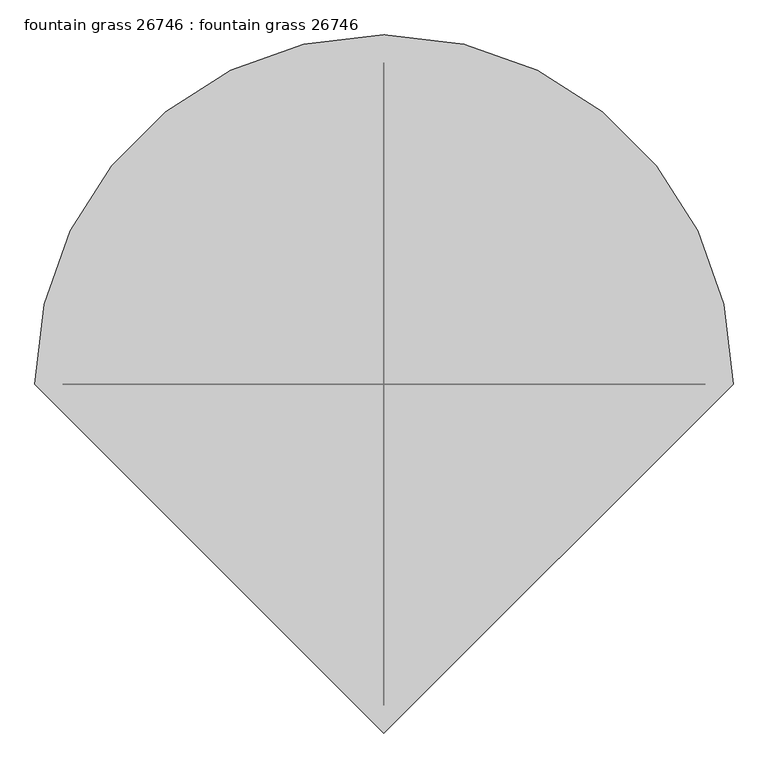
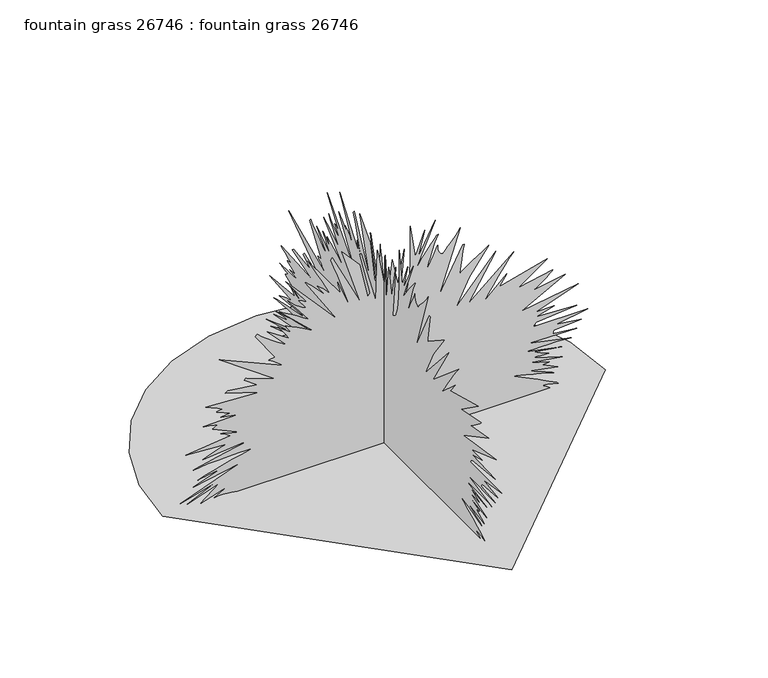
"""IFC4 building model written with IfcOpenShell, lengths in millimetres: proxy geometry, fountain grass 26746 : fountain grass 26746."""

from ifc_helpers import new_model, si_unit, origin, place, context, project, spatial, triangles, source, transform, mapped, element, save


def fountain_grass_26746_fountain_grass_26746_7c509b90(model_context):
    return source(origin(), model_context, "Body", "Tessellation", [
        triangles([(-1075.1021822, 0.0, 0.0), (-1046.6796438, 246.3421583, 0.0), (-965.7324045, 472.5690837, 0.0), (-838.7452429, 672.1950891, 0.0), (-672.1950891, 838.7452429, 0.0), (-472.5690837, 965.7324045, 0.0), (-246.341904, 1046.6796438, 0.0), (4.7e-05, 1075.1021822, 0.0), (246.3421583, 1046.6796438, 0.0), (472.5690837, 965.7324045, 0.0), (672.1950891, 838.7452429, 0.0), (838.7452429, 672.1950891, 0.0), (965.7324045, 472.5690837, 0.0), (1046.6796438, 246.341904, 0.0), (1075.1021822, -9.4e-05, 0.0), (-0.000141, -1075.1021822, 0.0), (-0.0002094, -151.7493584, 903.5253731), (-0.0002064, -197.8505688, 1023.5783649), (-0.0002098, -163.2745906, 893.9190554), (-0.000206, -247.7932689, 1057.1952084), (-0.0002115, -151.7493584, 831.4910345), (-0.0002109, -167.7051159, 857.3634378), (-0.0002104, -186.8993659, 885.4837418), (-0.0002098, -207.3806375, 913.5837708), (-0.0002093, -227.1984504, 939.3926605), (-0.0002089, -244.4013429, 960.6372213), (-0.0002086, -257.0401245, 975.0516758), (-0.0002085, -263.1615169, 980.3602907), (-0.0002094, -247.7267213, 943.5176268), (-0.0002103, -234.4486256, 908.2090988), (-0.0002111, -223.4664289, 876.1391087), (-0.0002118, -214.9206206, 848.9967247), (-0.0002123, -208.9511085, 828.4836599), (-0.0002127, -205.6989088, 816.294215), (-0.0002127, -205.3039292, 814.1250887), (-0.0002127, -208.3029104, 818.0239786), (-0.0002124, -216.0537091, 832.5501995), (-0.000212, -226.6881618, 853.6500017), (-0.0002116, -238.3378685, 877.271961), (-0.0002112, -249.1338665, 899.3648712), (-0.0002109, -257.207756, 915.8748373), (-0.0002107, -260.692645, 922.748037), (-0.0002103, -260.2582965, 906.3549242), (-0.0002103, -263.0522939, 893.568568), (-0.0002106, -267.949415, 883.9953152), (-0.0002111, -273.8345936, 877.2388962), (-0.0002116, -279.5876763, 872.9031143), (-0.000212, -284.0860209, 870.5917728), (-0.0002121, -286.2119994, 869.908457), (-0.0002118, -297.8807457, 886.1644415), (-0.0002115, -309.7933362, 900.0811066), (-0.0002113, -321.8837319, 912.8293837), (-0.0002111, -334.0884012, 925.5801315), (-0.0002109, -346.3388163, 939.504427), (-0.0002105, -358.5765141, 955.7731287), (-0.0002101, -370.7304234, 975.5571682), (-0.0002182, -267.0019983, 658.6111799), (-0.000213, -382.2543929, 884.3153538), (-0.0002131, -389.9378629, 884.3153538), (-0.0002137, -385.7570498, 861.6865025), (-0.0002144, -381.2002785, 835.410272), (-0.0002152, -376.6689054, 808.0824343), (-0.0002159, -372.5719171, 782.3039932), (-0.0002165, -369.305474, 760.6733368), (-0.0002169, -367.2760194, 745.7889982), (-0.0002171, -366.8873803, 740.2492201), (-0.0002169, -377.1819918, 749.4998909), (-0.0002168, -398.429096, 764.5798571), (-0.0002166, -426.0591682, 782.8856438), (-0.0002164, -455.5053723, 801.8137035), (-0.0002163, -482.19564, 818.763105), (-0.0002161, -501.5631351, 831.122743), (-0.0002161, -509.0332824, 836.294157), (-0.0002187, -412.9883454, 706.6349201), (-0.0002218, -347.6799408, 572.1725244), (-0.0002178, -543.6077345, 793.0735394), (-0.0002226, -409.1478822, 572.1725244), (-0.0002221, -630.0006443, 760.9578398), (-0.0002225, -607.1482965, 733.4877869), (-0.0002229, -581.7076618, 698.9640947), (-0.0002232, -555.6879564, 661.3112331), (-0.0002235, -531.0982146, 624.4456781), (-0.0002238, -509.9451453, 592.2867763), (-0.000224, -494.2377829, 568.7536923), (-0.0002241, -485.9827998, 557.7656639), (-0.0002226, -597.394713, 658.6111799), (-0.0002236, -558.9747108, 605.7868607), (-0.0002249, -793.3225067, 668.217425), (-0.000226, -651.1791481, 567.3694018), (-0.0002272, -820.215996, 600.9862453), (-0.0002273, -814.2901949, 595.3652584), (-0.0002274, -803.8635057, 586.2314046), (-0.0002276, -790.0737951, 574.7607748), (-0.0002278, -774.0693214, 562.1243005), (-0.0002279, -756.9878059, 549.4928767), (-0.000228, -739.9748909, 538.045138), (-0.0002281, -724.171059, 528.951943), (-0.0002293, -881.683901, 557.7656639), (-0.0002299, -666.5461607, 442.5132874), (-0.0002323, -943.1518787, 485.7338688), (-0.0002317, -735.6975357, 413.6995302), (-0.0002329, -827.8994659, 413.6995302), (-0.0002325, -739.5380716, 389.6889682), (-0.0002353, -935.4683361, 380.0852303), (-0.0002333, -739.5380716, 360.875211), (-0.0002334, -737.0615513, 358.3860097), (-0.0002334, -734.2345436, 355.2567312), (-0.0002335, -731.3236748, 351.8201314), (-0.0002335, -728.5931728, 348.4089297), (-0.0002336, -726.3148235, 345.3558457), (-0.0002336, -724.7527096, 342.9987222), (-0.0002337, -724.171059, 341.6677714), (-0.0002372, -989.2528439, 341.6677714), (-0.0002359, -835.5829359, 317.6571731), (-0.0002381, -958.5188187, 298.4471538), (-0.0002366, -824.0564592, 288.843434), (-0.000237, -820.215996, 274.4365736), (-0.0002389, -935.4683361, 260.0296949), (-0.0002357, -704.9635832, 264.8328356), (-0.0002397, -908.5748468, 221.6119818), (-0.0002392, -879.3065025, 224.4689658), (-0.0002387, -841.8263048, 226.3310433), (-0.0002381, -800.7671831, 227.3607588), (-0.0002376, -760.7622849, 227.7214381), (-0.0002371, -726.4494083, 227.5753896), (-0.0002368, -702.461701, 227.0854304), (-0.0002367, -693.4371065, 226.4143594), (-0.0002399, -862.4738817, 192.7990239), (-0.0002375, -720.3305958, 212.0077533), (-0.0002395, -801.079664, 180.0418811), (-0.0002393, -789.8198135, 180.8544223), (-0.0002391, -775.0700598, 181.8744909), (-0.0002389, -758.976638, 182.9049694), (-0.0002386, -743.6934866, 183.7490131), (-0.0002385, -731.3642973, 184.2100133), (-0.0002384, -724.1406103, 184.090889), (-0.0002384, -724.171059, 183.194523), (-0.0002416, -866.3169611, 139.9746865), (-0.0002388, -708.8040464, 163.9857935), (-0.0002409, -802.8830423, 135.5523002), (-0.0002408, -799.4514931, 134.831959), (-0.0002408, -794.1606823, 134.0915427), (-0.0002407, -787.8817778, 133.3391994), (-0.0002407, -781.4835491, 132.5827867), (-0.0002406, -775.8346207, 131.8306978), (-0.0002406, -771.8087036, 131.0902815), (-0.0002406, -770.2720242, 130.3701946), (-0.0002426, -843.2664785, 96.75485), (-0.0002398, -697.2953739, 122.86552), (-0.0002401, -707.9455233, 119.2147799), (-0.0002406, -727.4654074, 112.0362392), (-0.0002412, -752.0246641, 102.744419), (-0.0002418, -777.7954748, 92.7543584), (-0.0002424, -800.9424631, 83.4810781), (-0.0002428, -817.6404264, 76.3393719), (-0.000243, -824.0564592, 72.7440018), (-0.0002423, -793.2310152, 81.617738), (-0.0002416, -757.9402914, 91.2158803), (-0.0002408, -721.5396063, 100.7012479), (-0.0002401, -687.3868217, 109.2361467), (-0.0002395, -658.8372562, 115.9836545), (-0.0002392, -639.2462282, 120.1060682), (-0.000239, -631.9691288, 120.7659571), (-0.00024, -666.4089598, 103.8820858), (-0.0002411, -705.799288, 84.5753155), (-0.0002422, -746.4087278, 64.5205076), (-0.0002433, -784.498554, 45.3925509), (-0.0002442, -816.3297506, 28.8660546), (-0.0002449, -838.1686792, 16.6156986), (-0.0002452, -846.2788673, 10.3164533), (-0.0002449, -834.4653442, 14.1385651), (-0.0002446, -820.7849293, 17.3725156), (-0.0002444, -806.5482256, 20.018432), (-0.0002441, -793.0684525, 22.0761847), (-0.0002439, -781.6562857, 23.5461577), (-0.0002438, -773.6197123, 24.4280193), (-0.0002437, -770.2720242, 24.7219217), (-0.0002438, -772.6468792, 22.8719915), (-0.000244, -777.9732983, 19.2397436), (-0.0002442, -785.103023, 14.5784422), (-0.0002445, -792.8881582, 9.6414491), (-0.0002447, -800.1804457, 5.1824076), (-0.0002449, -805.8319902, 1.9544036), (-0.000245, -808.6894466, 0.7109504), (-0.0002248, 712.2762182, 7.55e-05), (-0.0002247, 716.251339, 1.888295), (-0.0002245, 727.0437761, 4.4398649), (-0.0002242, 742.9644613, 7.0367071), (-0.0002239, 762.3193119, 9.0605264), (-0.0002236, 783.416498, 9.8934675), (-0.0002233, 804.5594662, 8.9170168), (-0.0002232, 824.0564592, 5.5131917), (-0.0002229, 758.7480183, 43.9307805), (-0.0002224, 893.2079069, 0.7110012), (-0.0002215, 801.0059767, 72.7440018), (-0.000221, 954.6783554, 19.9198029), (-0.000221, 820.215996, 82.3482439), (-0.0002201, 989.2528439, 34.3262887), (-0.0002208, 701.1205765, 139.9746865), (-0.0002191, 927.7848661, 96.75485), (-0.0002194, 808.6894466, 139.9746865), (-0.0002193, 812.3292681, 139.9878942), (-0.0002192, 822.1235104, 138.9035673), (-0.0002191, 836.3982931, 136.9663127), (-0.000219, 853.4747217, 134.4199656), (-0.0002188, 871.6762997, 131.5086244), (-0.0002187, 889.3216616, 128.4766238), (-0.0002185, 904.7343836, 125.5680804), (-0.0002186, 893.5940025, 129.4418265), (-0.0002187, 867.1881289, 137.4656826), (-0.0002189, 829.5479118, 148.2962261), (-0.0002191, 784.7068262, 160.5885445), (-0.0002194, 736.7034336, 172.9992332), (-0.0002196, 689.5686653, 184.1843608), (-0.0002199, 647.3361414, 192.7990239), (-0.0002198, 647.3361414, 197.6011291), (-0.0002195, 670.2748575, 197.8660475), (-0.000219, 707.9862185, 197.3700022), (-0.0002184, 755.0320387, 196.1048178), (-0.0002178, 805.9742054, 194.0624097), (-0.0002172, 855.3746058, 191.2351477), (-0.0002168, 897.79004, 187.6151289), (-0.0002165, 927.7848661, 183.194523), (-0.0002165, 918.4681383, 186.3568118), (-0.0002167, 893.3831142, 192.5249491), (-0.0002169, 856.8325836, 200.7720656), (-0.0002172, 813.1090897, 210.171837), (-0.0002176, 766.5153494, 219.7974123), (-0.0002179, 721.3516817, 228.7219402), (-0.0002182, 681.9131006, 236.0185879), (-0.0002181, 681.9131006, 240.8209655), (-0.000216, 881.683901, 221.6119818), (-0.000216, 877.2592438, 223.6533724), (-0.000216, 864.5567488, 228.9396232), (-0.000216, 846.1366522, 236.2129074), (-0.0002161, 824.5568647, 244.2159255), (-0.0002161, 802.3750065, 251.6913958), (-0.0002162, 782.1465174, 257.3830178), (-0.0002164, 766.4315609, 260.0296949), (-0.0002133, 962.3618254, 274.4365736), (-0.0002155, 747.2215416, 298.4471538), (-0.0002154, 748.9690367, 300.212453), (-0.0002152, 753.6680231, 303.7532252), (-0.000215, 760.5209478, 308.3607565), (-0.0002147, 768.7124537, 313.3315287), (-0.0002145, 777.4449875, 317.9594075), (-0.0002143, 785.9107498, 321.5357517), (-0.0002141, 793.3021591, 323.3569342), (-0.0002142, 787.9021254, 322.9682951), (-0.0002145, 773.9448378, 319.7958507), (-0.0002149, 754.7907017, 314.8758748), (-0.0002153, 733.8001951, 309.2421344), (-0.0002157, 714.3387377, 303.9360992), (-0.0002161, 699.7641912, 299.9914817), (-0.0002162, 693.4371065, 298.4471538), (-0.0002125, 831.7399292, 360.875211), (-0.0002125, 830.7239302, 362.5795401), (-0.0002124, 827.9833271, 364.8223901), (-0.0002124, 823.9904022, 367.3496704), (-0.0002124, 819.2127142, 369.9125227), (-0.0002124, 814.1174583, 372.2544219), (-0.0002124, 809.1745914, 374.1289078), (-0.0002124, 804.8489834, 375.2820714), (-0.0002124, 807.681078, 376.3869822), (-0.0002122, 815.2883898, 378.2437366), (-0.000212, 826.3196205, 380.5906863), (-0.0002117, 839.4361164, 383.168763), (-0.0002115, 853.2892679, 385.7163909), (-0.0002112, 866.5404213, 387.9770087), (-0.000211, 877.8408943, 389.6889682), (-0.0002131, 712.6470531, 394.4920907), (-0.0002116, 793.3225067, 408.8989511), (-0.0002121, 743.3810783, 413.6995302), (-0.0002103, 812.5324533, 442.5132874), (-0.0002103, 811.3640654, 443.8569191), (-0.0002103, 808.2246494, 445.132023), (-0.0002103, 803.6476032, 446.2470712), (-0.0002104, 798.178969, 447.1106812), (-0.0002104, 792.3547606, 447.6364486), (-0.0002105, 786.7133898, 447.7354978), (-0.0002106, 781.7985008, 447.31641), (-0.0002105, 785.3392731, 449.5770278), (-0.0002102, 794.7525066, 454.4588882), (-0.0002098, 808.222106, 461.0349403), (-0.0002094, 823.9294321, 468.375517), (-0.000209, 840.0584621, 475.5561107), (-0.0002086, 854.7929552, 481.6521049), (-0.0002083, 866.3169611, 485.7338688), (-0.0002122, 605.078183, 471.3270083), (-0.0002084, 770.2720242, 524.1513276), (-0.0002083, 758.7480183, 533.7550655), (-0.0002108, 616.6021889, 514.5450826), (-0.0002087, 678.0700939, 557.7656639), (-0.0002085, 670.386624, 567.3694018), (-0.0002119, 528.2407219, 514.5450826), (-0.0002026, 801.0059767, 706.6349201), (-0.0002107, 493.6662698, 572.1725244), (-0.0002103, 502.7518707, 579.84077), (-0.0002099, 513.8160936, 588.6494983), (-0.0002095, 525.7210719, 597.7502872), (-0.0002091, 537.32883, 606.3024905), (-0.0002087, 547.4989941, 613.4576134), (-0.0002085, 555.0935886, 618.3700315), (-0.0002084, 558.9772542, 620.1936848), (-0.0002084, 557.3414892, 621.3672323), (-0.0002084, 553.1149303, 622.2358566), (-0.0002085, 547.2958088, 622.8886511), (-0.0002085, 540.8924569, 623.4067881), (-0.0002086, 534.9133161, 623.8742014), (-0.0002086, 530.3616317, 624.3770777), (-0.0002086, 528.2407219, 624.99688), (-0.0002032, 624.2856588, 764.2598185), (-0.000203, 616.6021889, 773.8661362), (-0.0002039, 593.2849711, 753.716276), (-0.0002049, 567.5725871, 733.8154558), (-0.0002058, 541.6163589, 715.1616526), (-0.0002066, 517.5625946, 698.7558226), (-0.0002072, 497.5601091, 685.596088), (-0.0002077, 483.7552105, 676.68326), (-0.0002079, 478.2992935, 673.0180767), (-0.0002038, 566.6607242, 769.062941), (-0.0002074, 459.0893106, 697.0286751), (-0.0002072, 461.8096387, 701.9384771), (-0.0002069, 466.5873631, 709.5711508), (-0.0002066, 473.2904423, 719.5050648), (-0.0002061, 481.786726, 731.3211313), (-0.0002056, 491.9467163, 744.6002626), (-0.000205, 503.6332486, 758.9207548), (-0.0002044, 516.7167523, 773.8661362), (-0.0002045, 513.2318996, 772.2836746), (-0.0002048, 504.2098123, 766.0124004), (-0.0002052, 491.8044648, 756.8075117), (-0.0002057, 478.1697593, 746.4290754), (-0.0002062, 465.4570905, 736.6373766), (-0.0002065, 455.8177806, 729.1875406), (-0.0002067, 451.4058043, 725.842396), (-0.0002064, 455.2462675, 731.5675552), (-0.0002062, 459.8665524, 738.7150841), (-0.0002059, 464.8017526, 746.5230377), (-0.0002056, 469.5794769, 754.2243118), (-0.0002053, 473.7349282, 761.0594324), (-0.0002051, 476.7956062, 766.2588243), (-0.000205, 478.2992935, 769.062941), (-0.0002053, 467.4382559, 763.1752916), (-0.0002059, 448.0021966, 753.3581583), (-0.0002066, 423.3616948, 740.947724), (-0.0002073, 396.8746124, 727.2876566), (-0.0002081, 371.9089851, 713.7214788), (-0.0002087, 351.8277617, 701.5879171), (-0.0002091, 339.9964345, 692.2280233), (-0.0002022, 509.0332824, 850.7010538), (-0.0002024, 501.3497761, 846.621797), (-0.000203, 481.4362023, 834.9479456), (-0.0002039, 453.9940547, 818.4430664), (-0.0002048, 423.7299863, 799.8731243), (-0.0002057, 395.3480704, 782.0093164), (-0.0002064, 373.5523441, 767.6151369), (-0.0002068, 363.0469171, 759.4592394), (-0.0002065, 368.546, 766.7414257), (-0.0002058, 383.526917, 785.5628059), (-0.0002047, 404.1618493, 811.3869564), (-0.0002036, 426.6281379, 839.67491), (-0.0002025, 447.1030509, 865.8851561), (-0.0002018, 461.7588424, 885.4786549), (-0.0002014, 466.7727805, 893.9190554), (-0.0002023, 448.2638449, 874.4677717), (-0.000203, 430.4813184, 858.5800787), (-0.0002036, 414.1669072, 846.0858559), (-0.000204, 400.0597741, 836.8173809), (-0.0002044, 388.9066395, 830.6070768), (-0.0002046, 381.4441226, 827.2873667), (-0.0002046, 378.4138933, 826.687912), (-0.0002027, 412.9883454, 874.7116522), (-0.0002028, 410.1994168, 874.6379648), (-0.0002029, 404.7105077, 872.2808413), (-0.0002031, 397.603565, 868.4733702), (-0.0002034, 389.9581741, 864.0537998), (-0.0002036, 382.8487244, 859.8627766), (-0.0002037, 377.3623587, 856.730991), (-0.0002038, 374.5708866, 855.5016329), (-0.0001983, 478.2992935, 994.7671148), (-0.0002099, 228.5847938, 716.2386217), (-0.0002007, 382.2543929, 956.3471489), (-0.0002008, 377.5401458, 953.682704), (-0.0002013, 366.727361, 944.1653343), (-0.0002019, 351.5610629, 929.5552523), (-0.0002027, 333.7912173, 911.6203005), (-0.0002035, 315.1705153, 892.1258509), (-0.0002043, 297.4463973, 872.8294996), (-0.000205, 282.3689745, 855.5016329), (-0.0002026, 324.6294582, 917.9296537), (-0.0002027, 320.6416566, 916.0831095), (-0.000203, 312.1021706, 909.1260487), (-0.0002035, 300.8906456, 898.981319), (-0.000204, 288.8891434, 887.5817968), (-0.0002045, 277.9849398, 876.8528732), (-0.0002048, 270.0626945, 868.7172506), (-0.000205, 267.0019983, 865.1053345), (-0.0002046, 271.2920526, 874.9732641), (-0.0002037, 283.4510124, 899.7559811), (-0.0002024, 300.8601605, 934.157733), (-0.000201, 320.9083554, 972.880006), (-0.0001996, 340.9768616, 1010.6243591), (-0.0001985, 358.4571536, 1042.097438), (-0.0001977, 370.7304234, 1061.9957874), (-0.0002064, 209.3757919, 841.0947361), (-0.0002061, 212.3376932, 849.9161453), (-0.0002058, 215.4885547, 860.5994322), (-0.0002054, 218.5616956, 872.0446638), (-0.000205, 221.2901628, 883.1571396), (-0.0002047, 223.4082747, 892.8396154), (-0.0002045, 224.6477885, 899.9947746), (-0.0002044, 224.7430407, 903.5253731), (-0.0002098, 163.2748449, 749.8529943), (-0.0002094, 166.4719427, 760.9984623), (-0.0002084, 175.9733068, 790.7926466), (-0.0002069, 190.101278, 833.7744707), (-0.0002052, 207.1779428, 884.4830034), (-0.0002033, 225.5248425, 937.4622551), (-0.0002016, 243.4645905, 987.2487511), (-0.0002002, 259.318492, 1028.3814875), (-0.0002, 251.6352582, 1037.9851891), (-0.0002099, 116.1998023, 765.6542828), (-0.0002002, 205.5340569, 1052.3920858), (-0.0002042, 117.1738889, 956.3471489), (-0.00021, 78.7561757, 778.6667152), (-0.00021, 77.3934682, 780.4573763), (-0.0002099, 75.5994689, 782.9009045), (-0.0002099, 73.577631, 785.6593117), (-0.0002098, 71.5275972, 788.3949005), (-0.0002098, 69.6525708, 790.7697556), (-0.0002097, 68.1529576, 792.4410925), (-0.0002097, 67.2306846, 793.0735394), (-0.0002026, 117.1738889, 1009.1714682), (-0.0002027, 109.4901464, 1009.1714682), (-0.0002115, 40.3384626, 745.0523426), (-0.000204, 32.6549699, 999.5677666), (-0.0002043, 30.2686421, 991.1984373), (-0.0002051, 25.7212838, 968.6636209), (-0.0002061, 19.6890689, 935.823983), (-0.0002074, 12.8482471, 896.5454212), (-0.0002087, 5.8757252, 854.6837322), (-0.00021, -0.5533969, 814.1047411), (-0.0002111, -5.7626445, 778.6667152), (-0.0002057, -5.7626445, 961.1502714), (-0.0002127, -17.2877302, 730.6455185), (-0.0002072, -40.3384626, 927.5359715), (-0.0002115, -67.2306846, 793.0735394), (-0.0002069, -97.9646508, 961.1502714), (-0.0002145, -74.9141773, 697.0286751), (-0.0002143, -99.6672177, 714.3946209), (-0.0002131, -115.3773507, 759.9418407), (-0.0002114, -124.0562722, 823.853274), (-0.0002092, -127.7161506, 896.3143307), (-0.0002071, -128.3684273, 967.5027906), (-0.0002053, -128.0255249, 1027.6042093), (-0.0002042, -128.6986215, 1066.79891), (151.7493584, 7.84e-05, 903.5253731), (197.8503144, 8.55e-05, 1023.5783649), (163.2745906, 7.78e-05, 893.9190554), (247.7932689, 8.75e-05, 1057.1952084), (151.7493584, 7.41e-05, 831.4910345), (167.7048616, 7.56e-05, 857.3634378), (186.8991115, 7.73e-05, 885.4837418), (207.3803832, 7.9e-05, 913.5837708), (227.1984504, 8.05e-05, 939.3901171), (244.4013429, 8.18e-05, 960.6372213), (257.0401245, 8.26e-05, 975.0516758), (263.1615169, 8.29e-05, 980.3602907), (247.726467, 8.07e-05, 943.5176268), (234.4483712, 7.86e-05, 908.2090988), (223.4661746, 7.67e-05, 876.1391087), (214.9203662, 7.51e-05, 848.9967247), (208.9508542, 7.39e-05, 828.4811165), (205.6986544, 7.32e-05, 816.294215), (205.3036749, 7.3e-05, 814.1250887), (208.3026561, 7.32e-05, 818.0239786), (216.0534548, 7.4e-05, 832.5501995), (226.6879074, 7.52e-05, 853.6500017), (238.3376142, 7.65e-05, 877.271961), (249.1336122, 7.77e-05, 899.3623278), (257.207756, 7.86e-05, 915.8748373), (260.692645, 7.9e-05, 922.748037), (260.2582965, 7.89e-05, 906.3549242), (263.0522939, 7.86e-05, 893.568568), (267.949415, 7.8e-05, 883.9953152), (273.8345936, 7.75e-05, 877.2388962), (279.5876763, 7.69e-05, 872.9031143), (284.0860209, 7.65e-05, 870.5917728), (286.2119994, 7.64e-05, 869.908457), (297.8807457, 7.73e-05, 886.1644415), (309.7933362, 7.82e-05, 900.0811066), (321.8837319, 7.89e-05, 912.8293837), (334.0884012, 7.97e-05, 925.5801315), (346.3388163, 8.05e-05, 939.504427), (358.5765141, 8.15e-05, 955.7731287), (370.7304234, 8.27e-05, 975.5571682), (267.0019983, 6.38e-05, 658.6111799), (382.2543929, 7.72e-05, 884.3153538), (389.9378629, 7.72e-05, 884.3153538), (385.7570498, 7.59e-05, 861.6865025), (381.2002785, 7.43e-05, 835.410272), (376.6689054, 7.27e-05, 808.0824343), (372.5693736, 7.11e-05, 782.3039932), (369.305474, 6.98e-05, 760.6733368), (367.2760194, 6.9e-05, 745.7889982), (366.8873803, 6.86e-05, 740.2492201), (377.1819918, 6.92e-05, 749.4998909), (398.429096, 7.01e-05, 764.5798571), (426.0591682, 7.12e-05, 782.8856438), (455.5053723, 7.23e-05, 801.8137035), (482.19564, 7.33e-05, 818.763105), (501.5631351, 7.4e-05, 831.122743), (509.0332824, 7.43e-05, 836.294157), (412.9883454, 6.66e-05, 706.6349201), (347.6799408, 5.86e-05, 572.1725244), (543.6077345, 7.18e-05, 793.0735394), (409.1478822, 5.86e-05, 572.1725244), (629.9981009, 6.77e-05, 760.9578398), (607.145753, 6.62e-05, 733.4877869), (581.7076618, 6.44e-05, 698.9640947), (555.6879564, 6.26e-05, 661.3112331), (531.0982146, 6.09e-05, 624.4456781), (509.9451453, 5.94e-05, 592.2867763), (494.2377829, 5.83e-05, 568.7536923), (485.9827998, 5.77e-05, 557.7656639), (597.3921696, 6.38e-05, 658.6111799), (558.9747108, 6.06e-05, 605.7868607), (793.3225067, 6.43e-05, 668.217425), (651.1791481, 5.83e-05, 567.3694018), (820.215996, 6.03e-05, 600.9862453), (814.2901949, 6e-05, 595.3652584), (803.8635057, 5.94e-05, 586.2314046), (790.0737951, 5.88e-05, 574.7607748), (774.0693214, 5.8e-05, 562.1243005), (756.9878059, 5.73e-05, 549.4928767), (739.9748909, 5.66e-05, 538.045138), (724.171059, 5.6e-05, 528.951943), (881.683901, 5.77e-05, 557.7656639), (666.5461607, 5.09e-05, 442.5132874), (943.1518787, 5.35e-05, 485.7338688), (735.6975357, 4.92e-05, 413.6995302), (827.8994659, 4.92e-05, 413.6995302), (739.5380716, 4.77e-05, 389.6889682), (935.4683361, 4.72e-05, 380.0852303), (739.5380716, 4.6e-05, 360.875211), (737.0615513, 4.59e-05, 358.3860097), (734.2345436, 4.57e-05, 355.2567312), (731.3236748, 4.55e-05, 351.8201314), (728.5931728, 4.53e-05, 348.4089297), (726.3148235, 4.51e-05, 345.3558457), (724.7527096, 4.49e-05, 342.9987222), (724.171059, 4.49e-05, 341.6677714), (989.2528439, 4.49e-05, 341.6677714), (835.5829359, 4.34e-05, 317.6571731), (958.5188187, 4.23e-05, 298.4471538), (824.0564592, 4.17e-05, 288.843434), (820.215996, 4.09e-05, 274.4365736), (935.4683361, 4e-05, 260.0296949), (704.9635832, 4.03e-05, 264.8328356), (908.5748468, 3.77e-05, 221.6119818), (879.3065025, 3.79e-05, 224.4689658), (841.8263048, 3.8e-05, 226.3310433), (800.7647123, 3.81e-05, 227.3607588), (760.7622849, 3.81e-05, 227.7211837), (726.4494083, 3.81e-05, 227.5753896), (702.461701, 3.8e-05, 227.0854304), (693.4371065, 3.8e-05, 226.4141051), (862.4738817, 3.6e-05, 192.7987696), (720.3305958, 3.71e-05, 212.007499), (801.079664, 3.52e-05, 180.0418811), (789.8198135, 3.53e-05, 180.8544223), (775.0700598, 3.53e-05, 181.8744909), (758.976638, 3.54e-05, 182.9049694), (743.6934866, 3.55e-05, 183.7490131), (731.3642973, 3.55e-05, 184.2100133), (724.1406103, 3.55e-05, 184.090889), (724.171059, 3.54e-05, 183.194523), (866.3169611, 3.28e-05, 139.9746865), (708.8040464, 3.43e-05, 163.9857935), (802.8830423, 3.26e-05, 135.5523002), (799.4514931, 3.25e-05, 134.831959), (794.1606823, 3.25e-05, 134.0915427), (787.8817778, 3.24e-05, 133.3391994), (781.4810057, 3.24e-05, 132.5827867), (775.8346207, 3.24e-05, 131.8306978), (771.8087036, 3.23e-05, 131.0902815), (770.2720242, 3.23e-05, 130.3701946), (843.2664785, 3.03e-05, 96.75485), (697.2953739, 3.18e-05, 122.8652657), (707.9455233, 3.16e-05, 119.2147799), (727.4654074, 3.12e-05, 112.0362392), (752.0246641, 3.06e-05, 102.744419), (777.7954748, 3e-05, 92.7543584), (800.9424631, 2.95e-05, 83.4810781), (817.6404264, 2.91e-05, 76.3393719), (824.0564592, 2.88e-05, 72.7440018), (793.2310152, 2.94e-05, 81.617738), (757.9402914, 2.99e-05, 91.2158803), (721.5396063, 3.05e-05, 100.7012479), (687.3868217, 3.1e-05, 109.2361467), (658.8372562, 3.14e-05, 115.9836545), (639.2462282, 3.17e-05, 120.1060682), (631.9691288, 3.17e-05, 120.7659571), (666.4089598, 3.07e-05, 103.8820858), (705.799288, 2.95e-05, 84.5753155), (746.4087278, 2.83e-05, 64.5205076), (784.498554, 2.72e-05, 45.3925509), (816.3297506, 2.62e-05, 28.8660546), (838.1686792, 2.55e-05, 16.6156986), (846.2788673, 2.51e-05, 10.3164533), (834.4653442, 2.53e-05, 14.1385651), (820.7849293, 2.55e-05, 17.3724907), (806.5482256, 2.57e-05, 20.018432), (793.0684525, 2.58e-05, 22.0761598), (781.6562857, 2.59e-05, 23.5461577), (773.6197123, 2.6e-05, 24.4280193), (770.2720242, 2.6e-05, 24.7219217), (772.6468792, 2.59e-05, 22.8719915), (777.9732983, 2.56e-05, 19.2397436), (785.103023, 2.54e-05, 14.5784422), (792.8881582, 2.51e-05, 9.6414491), (800.1804457, 2.48e-05, 5.1824076), (805.8319902, 2.46e-05, 1.9544036), (808.6894466, 2.45e-05, 0.7109504), (-712.2762182, 2.45e-05, 3.05e-05), (-716.251339, 2.46e-05, 1.8882493), (-727.0437761, 2.48e-05, 4.4398141), (-742.9644613, 2.49e-05, 7.0366566), (-762.3193119, 2.5e-05, 9.0604759), (-783.416498, 2.51e-05, 9.8934175), (-804.5594662, 2.5e-05, 8.9169657), (-824.0564592, 2.48e-05, 5.5131406), (-758.7480183, 2.71e-05, 43.9307805), (-893.2104504, 2.45e-05, 0.7109504), (-801.0059767, 2.88e-05, 72.7440018), (-954.6783554, 2.57e-05, 19.919753), (-820.215996, 2.94e-05, 82.3482439), (-989.2528439, 2.65e-05, 34.3262887), (-701.1205765, 3.28e-05, 139.9746865), (-927.7848661, 3.03e-05, 96.75485), (-808.6894466, 3.28e-05, 139.9746865), (-812.3292681, 3.28e-05, 139.9878942), (-822.1235104, 3.28e-05, 138.9035673), (-836.3982931, 3.27e-05, 136.9663127), (-853.4747217, 3.25e-05, 134.4197112), (-871.6762997, 3.23e-05, 131.5086244), (-889.3216616, 3.22e-05, 128.4766238), (-904.7343836, 3.2e-05, 125.5680804), (-893.5940025, 3.22e-05, 129.4418265), (-867.1881289, 3.27e-05, 137.4656826), (-829.5479118, 3.33e-05, 148.2959718), (-784.7068262, 3.41e-05, 160.5885445), (-736.7034336, 3.48e-05, 172.9992332), (-689.5686653, 3.55e-05, 184.1841064), (-647.3361414, 3.6e-05, 192.7987696), (-647.3361414, 3.63e-05, 197.6011291), (-670.2748575, 3.63e-05, 197.8660475), (-707.9862185, 3.63e-05, 197.3700022), (-755.0320387, 3.62e-05, 196.1045634), (-805.9767488, 3.61e-05, 194.0621554), (-855.3746058, 3.59e-05, 191.2351477), (-897.79004, 3.57e-05, 187.6151289), (-927.7848661, 3.54e-05, 183.194523), (-918.4681383, 3.56e-05, 186.3568118), (-893.3831142, 3.6e-05, 192.5249491), (-856.8325836, 3.65e-05, 200.7720656), (-813.1090897, 3.7e-05, 210.1715827), (-766.5153494, 3.76e-05, 219.797158), (-721.3516817, 3.81e-05, 228.7216859), (-681.9131006, 3.86e-05, 236.0185879), (-681.9131006, 3.89e-05, 240.8207112), (-881.683901, 3.77e-05, 221.6119818), (-877.2592438, 3.78e-05, 223.6533724), (-864.5567488, 3.81e-05, 228.9396232), (-846.1391956, 3.86e-05, 236.2129074), (-824.5568647, 3.91e-05, 244.2156711), (-802.3750065, 3.95e-05, 251.6913958), (-782.1465174, 3.98e-05, 257.3804744), (-766.4315609, 4e-05, 260.0296949), (-962.3618254, 4.09e-05, 274.4365736), (-747.2215416, 4.23e-05, 298.4471538), (-748.9690367, 4.24e-05, 300.212453), (-753.6705666, 4.26e-05, 303.7532252), (-760.5209478, 4.29e-05, 308.3607565), (-768.7149971, 4.32e-05, 313.3315287), (-777.4475309, 4.35e-05, 317.9594075), (-785.9107498, 4.37e-05, 321.5357517), (-793.3021591, 4.38e-05, 323.3569342), (-787.9021254, 4.38e-05, 322.9682951), (-773.9448378, 4.36e-05, 319.7958507), (-754.7907017, 4.33e-05, 314.8758748), (-733.8001951, 4.29e-05, 309.2421344), (-714.3387377, 4.26e-05, 303.9360992), (-699.7641912, 4.24e-05, 299.9914817), (-693.4371065, 4.23e-05, 298.4471538), (-831.7399292, 4.6e-05, 360.875211), (-830.7239302, 4.61e-05, 362.5795401), (-827.9833271, 4.62e-05, 364.8223901), (-823.9929457, 4.64e-05, 367.3496704), (-819.2127142, 4.66e-05, 369.9099792), (-814.1174583, 4.67e-05, 372.2544219), (-809.1745914, 4.68e-05, 374.1289078), (-804.8489834, 4.69e-05, 375.2820714), (-807.681078, 4.69e-05, 376.3869822), (-815.2883898, 4.7e-05, 378.2437366), (-826.3196205, 4.72e-05, 380.5906863), (-839.4361164, 4.73e-05, 383.168763), (-853.2918114, 4.75e-05, 385.7163909), (-866.5404213, 4.76e-05, 387.9770087), (-877.8408943, 4.77e-05, 389.6889682), (-712.6470531, 4.8e-05, 394.4920907), (-793.3225067, 4.89e-05, 408.8989511), (-743.3810783, 4.92e-05, 413.6995302), (-812.5324533, 5.09e-05, 442.5132874), (-811.3640654, 5.1e-05, 443.8569191), (-808.2246494, 5.1e-05, 445.132023), (-803.6501467, 5.11e-05, 446.2445277), (-798.178969, 5.12e-05, 447.1106812), (-792.3547606, 5.12e-05, 447.6364486), (-786.7133898, 5.12e-05, 447.7354978), (-781.7985008, 5.12e-05, 447.31641), (-785.3392731, 5.13e-05, 449.5770278), (-794.7525066, 5.16e-05, 454.4588882), (-808.222106, 5.2e-05, 461.0349403), (-823.9294321, 5.24e-05, 468.375517), (-840.0584621, 5.28e-05, 475.5561107), (-854.7929552, 5.32e-05, 481.6521049), (-866.3169611, 5.35e-05, 485.7338688), (-605.078183, 5.26e-05, 471.3270083), (-770.2720242, 5.57e-05, 524.1513276), (-758.7480183, 5.63e-05, 533.7550655), (-616.6021889, 5.52e-05, 514.5450826), (-678.0700939, 5.77e-05, 557.7656639), (-670.386624, 5.83e-05, 567.3694018), (-528.2432653, 5.52e-05, 514.5450826), (-801.0059767, 6.66e-05, 706.6349201), (-493.6662698, 5.86e-05, 572.1725244), (-502.7518707, 5.91e-05, 579.84077), (-513.8160936, 5.96e-05, 588.6494983), (-525.7210719, 6.01e-05, 597.7502872), (-537.32883, 6.06e-05, 606.3024905), (-547.4989941, 6.11e-05, 613.4576134), (-555.0935886, 6.14e-05, 618.3700315), (-558.9772542, 6.15e-05, 620.1936848), (-557.3440327, 6.15e-05, 621.3672323), (-553.1149303, 6.16e-05, 622.2358566), (-547.2958088, 6.16e-05, 622.8886511), (-540.8924569, 6.17e-05, 623.4042446), (-534.9133161, 6.17e-05, 623.8742014), (-530.3616317, 6.17e-05, 624.3770777), (-528.2432653, 6.18e-05, 624.99688), (-624.2856588, 7.01e-05, 764.2598185), (-616.6021889, 7.06e-05, 773.8635927), (-593.2849711, 6.94e-05, 753.716276), (-567.5725871, 6.82e-05, 733.8154558), (-541.6163589, 6.71e-05, 715.1616526), (-517.5625946, 6.62e-05, 698.7558226), (-497.5601091, 6.54e-05, 685.596088), (-483.7552105, 6.48e-05, 676.68326), (-478.2992935, 6.46e-05, 673.0180767), (-566.6607242, 7.03e-05, 769.062941), (-459.091854, 6.6e-05, 697.0286751), (-461.8096387, 6.63e-05, 701.9384771), (-466.5873631, 6.68e-05, 709.5711508), (-473.2904423, 6.74e-05, 719.5050648), (-481.786726, 6.81e-05, 731.3211313), (-491.9467163, 6.89e-05, 744.6002626), (-503.6332486, 6.97e-05, 758.9207548), (-516.7167523, 7.06e-05, 773.8635927), (-513.2318996, 7.05e-05, 772.2836746), (-504.2098123, 7.02e-05, 766.0124004), (-491.8044648, 6.96e-05, 756.8075117), (-478.1697593, 6.9e-05, 746.4290754), (-465.4570905, 6.84e-05, 736.6373766), (-455.8177806, 6.8e-05, 729.1875406), (-451.4058043, 6.78e-05, 725.842396), (-455.2462675, 6.81e-05, 731.5675552), (-459.8665524, 6.85e-05, 738.7150841), (-464.8017526, 6.9e-05, 746.5230377), (-469.5794769, 6.95e-05, 754.2243118), (-473.7349282, 6.99e-05, 761.0594324), (-476.7981497, 7.02e-05, 766.2588243), (-478.2992935, 7.03e-05, 769.062941), (-467.4382559, 7e-05, 763.1752916), (-448.0021966, 6.94e-05, 753.3581583), (-423.3616948, 6.87e-05, 740.947724), (-396.8746124, 6.79e-05, 727.2876566), (-371.9089851, 6.7e-05, 713.7214788), (-351.8277617, 6.63e-05, 701.5879171), (-339.9964345, 6.58e-05, 692.2280233), (-509.0332824, 7.52e-05, 850.7010538), (-501.3497761, 7.5e-05, 846.621797), (-481.4362023, 7.43e-05, 834.9479456), (-453.9940547, 7.33e-05, 818.4430664), (-423.7299863, 7.22e-05, 799.8731243), (-395.3480704, 7.11e-05, 782.0093164), (-373.5523441, 7.03e-05, 767.6151369), (-363.0469171, 6.98e-05, 759.4592394), (-368.546, 7.02e-05, 766.7414257), (-383.526917, 7.13e-05, 785.5628059), (-404.1618493, 7.29e-05, 811.3869564), (-426.6281379, 7.46e-05, 839.67491), (-447.1030509, 7.61e-05, 865.8851561), (-461.7588424, 7.73e-05, 885.4786549), (-466.7727805, 7.78e-05, 893.9190554), (-448.2638449, 7.66e-05, 874.4677717), (-430.4813184, 7.57e-05, 858.5800787), (-414.1669072, 7.49e-05, 846.0858559), (-400.0623176, 7.44e-05, 836.8173809), (-388.9066395, 7.4e-05, 830.6070768), (-381.4441226, 7.38e-05, 827.2873667), (-378.4138933, 7.38e-05, 826.687912), (-412.9883454, 7.66e-05, 874.7116522), (-410.1994168, 7.66e-05, 874.6379648), (-404.7105077, 7.65e-05, 872.2808413), (-397.603565, 7.63e-05, 868.4733702), (-389.9581741, 7.6e-05, 864.0537998), (-382.8487244, 7.58e-05, 859.8627766), (-377.3623587, 7.56e-05, 856.730991), (-374.5708866, 7.55e-05, 855.5016329), (-478.2992935, 8.38e-05, 994.7671148), (-228.5850482, 6.72e-05, 716.2386217), (-382.2543929, 8.15e-05, 956.3471489), (-377.5401458, 8.13e-05, 953.682704), (-366.727361, 8.08e-05, 944.1653343), (-351.5610629, 7.99e-05, 929.5552523), (-333.7912173, 7.88e-05, 911.6203005), (-315.1730587, 7.77e-05, 892.1258509), (-297.4463973, 7.65e-05, 872.8294996), (-282.3689745, 7.55e-05, 855.5016329), (-324.6294582, 7.92e-05, 917.9296537), (-320.6442, 7.91e-05, 916.0831095), (-312.1021706, 7.87e-05, 909.1260487), (-300.8906456, 7.81e-05, 898.981319), (-288.8891434, 7.74e-05, 887.5817968), (-277.9874833, 7.68e-05, 876.8528732), (-270.0626945, 7.63e-05, 868.7172506), (-267.0019983, 7.61e-05, 865.1053345), (-271.2920526, 7.67e-05, 874.9732641), (-283.4510124, 7.81e-05, 899.7559811), (-300.8601605, 8.02e-05, 934.157733), (-320.9083554, 8.25e-05, 972.880006), (-340.9768616, 8.47e-05, 1010.6243591), (-358.4571536, 8.66e-05, 1042.097438), (-370.7304234, 8.78e-05, 1061.9957874), (-209.3760462, 7.46e-05, 841.0947361), (-212.3379476, 7.52e-05, 849.9161453), (-215.4885547, 7.58e-05, 860.5994322), (-218.5616956, 7.65e-05, 872.0446638), (-221.2904171, 7.71e-05, 883.1571396), (-223.4082747, 7.77e-05, 892.8396154), (-224.6480428, 7.81e-05, 899.9947746), (-224.7430407, 7.84e-05, 903.5253731), (-163.2750993, 6.92e-05, 749.8529943), (-166.4719427, 6.99e-05, 760.9984623), (-175.9735611, 7.16e-05, 790.7901031), (-190.1015323, 7.42e-05, 833.7719273), (-207.1779428, 7.72e-05, 884.4830034), (-225.5250968, 8.04e-05, 937.4622551), (-243.4648448, 8.33e-05, 987.2487511), (-259.318492, 8.58e-05, 1028.3814875), (-251.6355125, 8.64e-05, 1037.9851891), (-116.2000566, 7.01e-05, 765.6542828), (-205.5343112, 8.72e-05, 1052.3920858), (-117.1738889, 8.15e-05, 956.3471489), (-78.7564301, 7.09e-05, 778.6667152), (-77.3934682, 7.1e-05, 780.4573763), (-75.5999776, 7.12e-05, 782.9009045), (-73.5778853, 7.13e-05, 785.6593117), (-71.5278515, 7.15e-05, 788.3949005), (-69.6528251, 7.16e-05, 790.7697556), (-68.1529576, 7.17e-05, 792.4410925), (-67.2311933, 7.18e-05, 793.0735394), (-117.1738889, 8.47e-05, 1009.1714682), (-109.4904008, 8.47e-05, 1009.1714682), (-40.3384626, 6.89e-05, 745.0523426), (-32.6552242, 8.41e-05, 999.5677666), (-30.2688964, 8.36e-05, 991.1984373), (-25.7212838, 8.22e-05, 968.6636209), (-19.6892211, 8.03e-05, 935.823983), (-12.8484243, 7.79e-05, 896.5454212), (-5.8759029, 7.54e-05, 854.6837322), (0.5532267, 7.3e-05, 814.1047411), (5.7624668, 7.09e-05, 778.6667152), (5.7624668, 8.18e-05, 961.1502714), (17.2875781, 6.81e-05, 730.6455185), (40.3382082, 7.98e-05, 927.5359715), (67.2306846, 7.18e-05, 793.0735394), (97.9646508, 8.18e-05, 961.1502714), (74.9141773, 6.6e-05, 697.0286751), (99.6669633, 6.71e-05, 714.3946209), (115.3770963, 6.98e-05, 759.9418407), (124.0560179, 7.36e-05, 823.853274), (127.7158962, 7.79e-05, 896.3143307), (128.3679186, 8.22e-05, 967.5027906), (128.0250162, 8.58e-05, 1027.6042093), (128.6986215, 8.81e-05, 1066.79891)], [[16, 15, 1], [15, 14, 1], [1, 14, 2], [14, 13, 2], [2, 13, 3], [3, 13, 4], [13, 12, 4], [12, 11, 4], [4, 11, 5], [5, 11, 6], [6, 11, 7], [7, 11, 8], [8, 11, 9], [9, 11, 10], [128, 127, 129], [198, 197, 199], [445, 444, 446], [118, 117, 119], [405, 404, 406], [20, 19, 21], [196, 195, 197], [120, 119, 121], [381, 380, 382], [449, 448, 450], [138, 137, 139], [104, 103, 105], [208, 207, 209], [113, 112, 114], [18, 17, 19], [200, 199, 201], [248, 247, 249], [404, 403, 406], [121, 119, 122], [270, 269, 271], [100, 99, 101], [223, 222, 224], [224, 222, 225], [240, 239, 241], [78, 77, 79], [269, 268, 271], [296, 295, 297], [115, 114, 116], [403, 402, 406], [76, 75, 77], [156, 155, 157], [155, 154, 157], [268, 267, 271], [457, 456, 17], [122, 119, 123], [86, 85, 87], [148, 147, 149], [102, 101, 103], [272, 271, 273], [321, 320, 322], [267, 266, 271], [456, 455, 17], [288, 287, 289], [365, 364, 366], [402, 401, 406], [364, 363, 366], [351, 350, 352], [352, 350, 353], [353, 350, 354], [79, 77, 80], [130, 129, 131], [98, 97, 99], [266, 265, 271], [56, 55, 57], [354, 350, 355], [232, 231, 233], [233, 231, 234], [234, 231, 235], [235, 231, 236], [236, 231, 237], [287, 286, 289], [131, 129, 132], [237, 231, 238], [238, 231, 239], [123, 119, 124], [192, 191, 193], [170, 169, 171], [88, 87, 89], [194, 193, 195], [73, 72, 74], [265, 264, 271], [401, 400, 406], [80, 77, 81], [286, 285, 289], [355, 350, 356], [184, 183, 185], [249, 247, 250], [247, 246, 250], [132, 129, 133], [285, 284, 289], [72, 71, 74], [437, 436, 438], [438, 436, 439], [439, 436, 440], [440, 436, 441], [55, 54, 57], [447, 446, 448], [329, 328, 330], [330, 328, 331], [140, 139, 141], [141, 139, 142], [142, 139, 143], [143, 139, 144], [284, 283, 289], [209, 207, 210], [207, 206, 210], [81, 77, 82], [356, 350, 357], [441, 436, 442], [183, 182, 185], [413, 412, 414], [412, 411, 414], [411, 410, 414], [410, 409, 414], [409, 408, 414], [408, 407, 414], [407, 406, 414], [144, 139, 145], [455, 454, 17], [71, 70, 74], [264, 263, 271], [400, 399, 406], [182, 181, 185], [283, 282, 289], [383, 382, 384], [384, 382, 385], [385, 382, 386], [386, 382, 387], [387, 382, 388], [388, 382, 389], [389, 382, 390], [181, 180, 185], [28, 27, 29], [27, 26, 29], [424, 423, 425], [425, 423, 426], [180, 179, 185], [90, 89, 91], [91, 89, 92], [92, 89, 93], [124, 119, 125], [54, 53, 57], [133, 129, 134], [154, 153, 157], [157, 153, 158], [153, 152, 158], [357, 350, 358], [179, 178, 185], [191, 190, 193], [145, 139, 146], [391, 390, 392], [392, 390, 393], [393, 390, 394], [394, 390, 395], [93, 89, 94], [42, 41, 43], [82, 77, 83], [94, 89, 95], [282, 281, 289], [178, 177, 185], [442, 436, 443], [53, 52, 57], [343, 342, 344], [70, 69, 74], [52, 51, 57], [51, 50, 57], [50, 49, 57], [95, 89, 96], [395, 390, 396], [222, 221, 225], [225, 221, 226], [399, 398, 406], [342, 341, 344], [206, 205, 210], [210, 205, 211], [205, 204, 211], [96, 89, 97], [83, 77, 84], [134, 129, 135], [197, 195, 199], [146, 139, 147], [147, 139, 149], [366, 363, 367], [363, 362, 367], [367, 362, 368], [158, 152, 159], [152, 151, 159], [246, 245, 250], [250, 245, 251], [245, 244, 251], [204, 203, 211], [373, 372, 374], [374, 372, 375], [375, 372, 376], [376, 372, 377], [377, 372, 378], [443, 436, 444], [290, 289, 291], [291, 289, 292], [84, 77, 85], [190, 189, 193], [69, 68, 74], [304, 303, 305], [448, 446, 450], [169, 168, 171], [171, 168, 172], [41, 40, 43], [331, 328, 332], [328, 327, 332], [125, 119, 126], [172, 168, 173], [378, 372, 379], [305, 303, 306], [195, 193, 199], [211, 203, 212], [203, 202, 212], [202, 201, 212], [201, 199, 212], [212, 199, 213], [213, 199, 214], [168, 167, 173], [173, 167, 174], [26, 25, 29], [29, 25, 30], [174, 167, 175], [332, 327, 333], [327, 326, 333], [25, 24, 30], [274, 273, 275], [275, 273, 276], [276, 273, 277], [277, 273, 278], [278, 273, 279], [279, 273, 280], [280, 273, 281], [281, 273, 289], [273, 271, 289], [135, 129, 136], [396, 390, 397], [362, 361, 368], [368, 361, 369], [341, 340, 344], [239, 231, 241], [244, 243, 251], [251, 243, 252], [243, 242, 252], [242, 241, 252], [241, 231, 252], [252, 231, 253], [253, 231, 254], [254, 231, 255], [97, 89, 99], [379, 372, 380], [380, 372, 382], [256, 255, 257], [257, 255, 258], [258, 255, 259], [259, 255, 260], [260, 255, 261], [261, 255, 262], [262, 255, 263], [263, 255, 271], [114, 112, 116], [151, 150, 159], [159, 150, 160], [150, 149, 160], [434, 433, 435], [435, 433, 436], [293, 292, 294], [294, 292, 295], [292, 289, 295], [333, 326, 334], [326, 325, 334], [30, 24, 31], [24, 23, 31], [444, 436, 446], [422, 421, 423], [421, 420, 423], [420, 419, 423], [419, 418, 423], [418, 417, 423], [417, 416, 423], [416, 415, 423], [415, 414, 423], [59, 58, 60], [58, 57, 60], [60, 57, 61], [61, 57, 62], [62, 57, 63], [63, 57, 64], [64, 57, 65], [65, 57, 66], [369, 361, 370], [68, 67, 74], [43, 40, 44], [31, 23, 32], [23, 22, 32], [32, 22, 33], [344, 340, 345], [340, 339, 345], [339, 338, 345], [303, 302, 306], [306, 302, 307], [189, 188, 193], [334, 325, 335], [325, 324, 335], [226, 221, 227], [221, 220, 227], [227, 220, 228], [220, 219, 228], [228, 219, 229], [219, 218, 229], [229, 218, 230], [218, 217, 230], [361, 360, 370], [370, 360, 371], [371, 360, 372], [372, 360, 382], [360, 359, 382], [359, 358, 382], [358, 350, 382], [335, 324, 336], [324, 323, 336], [175, 167, 176], [167, 166, 176], [176, 166, 177], [177, 166, 185], [166, 165, 185], [165, 164, 185], [164, 163, 185], [312, 311, 313], [313, 311, 314], [314, 311, 315], [315, 311, 316], [316, 311, 317], [317, 311, 318], [116, 112, 117], [117, 112, 119], [318, 311, 319], [307, 302, 308], [302, 301, 308], [308, 301, 309], [338, 337, 345], [345, 337, 346], [337, 336, 346], [397, 390, 398], [390, 382, 398], [398, 382, 406], [406, 382, 414], [433, 432, 436], [432, 431, 436], [431, 430, 436], [430, 429, 436], [429, 428, 436], [428, 427, 436], [427, 426, 436], [49, 48, 57], [126, 119, 127], [22, 21, 33], [33, 21, 34], [34, 21, 35], [67, 66, 74], [74, 66, 75], [66, 57, 75], [40, 39, 44], [44, 39, 45], [309, 301, 310], [301, 300, 310], [310, 300, 311], [271, 255, 289], [48, 47, 57], [454, 453, 17], [17, 453, 19], [19, 453, 21], [319, 311, 320], [217, 216, 230], [453, 452, 21], [21, 452, 35], [193, 188, 199], [188, 187, 199], [187, 186, 199], [186, 185, 199], [185, 163, 199], [199, 163, 214], [214, 163, 215], [215, 163, 216], [323, 322, 336], [47, 46, 57], [89, 87, 99], [87, 85, 99], [101, 99, 103], [103, 99, 105], [105, 99, 106], [106, 99, 107], [107, 99, 108], [108, 99, 109], [109, 99, 110], [110, 99, 111], [111, 99, 112], [311, 300, 320], [300, 299, 320], [299, 298, 320], [298, 297, 320], [160, 149, 161], [149, 139, 161], [129, 127, 136], [112, 99, 119], [45, 39, 46], [46, 39, 57], [39, 38, 57], [38, 37, 57], [37, 36, 57], [36, 35, 57], [35, 452, 57], [452, 451, 57], [426, 423, 436], [230, 216, 231], [336, 322, 346], [346, 322, 347], [99, 85, 119], [119, 85, 127], [137, 136, 139], [136, 127, 139], [139, 127, 161], [161, 127, 162], [127, 85, 162], [162, 85, 163], [163, 85, 216], [85, 77, 216], [77, 75, 216], [75, 57, 216], [216, 57, 231], [231, 57, 255], [255, 57, 289], [289, 57, 295], [295, 57, 297], [297, 57, 320], [320, 57, 322], [347, 322, 348], [451, 450, 57], [348, 322, 349], [349, 322, 350], [322, 57, 350], [57, 450, 350], [350, 450, 382], [450, 446, 382], [446, 436, 382], [382, 436, 414], [436, 423, 414], [569, 568, 570], [639, 638, 640], [886, 885, 887], [559, 558, 560], [846, 845, 847], [461, 460, 462], [637, 636, 638], [561, 560, 562], [822, 821, 823], [890, 889, 891], [579, 578, 580], [545, 544, 546], [649, 648, 650], [554, 553, 555], [459, 458, 460], [641, 640, 642], [689, 688, 690], [845, 844, 847], [562, 560, 563], [711, 710, 712], [541, 540, 542], [664, 663, 665], [665, 663, 666], [681, 680, 682], [519, 518, 520], [710, 709, 712], [737, 736, 738], [556, 555, 557], [844, 843, 847], [517, 516, 518], [597, 596, 598], [596, 595, 598], [709, 708, 712], [898, 897, 458], [563, 560, 564], [527, 526, 528], [589, 588, 590], [543, 542, 544], [713, 712, 714], [762, 761, 763], [708, 707, 712], [897, 896, 458], [729, 728, 730], [806, 805, 807], [843, 842, 847], [805, 804, 807], [792, 791, 793], [793, 791, 794], [794, 791, 795], [520, 518, 521], [571, 570, 572], [539, 538, 540], [707, 706, 712], [497, 496, 498], [795, 791, 796], [673, 672, 674], [674, 672, 675], [675, 672, 676], [676, 672, 677], [677, 672, 678], [728, 727, 730], [572, 570, 573], [678, 672, 679], [679, 672, 680], [564, 560, 565], [633, 632, 634], [611, 610, 612], [529, 528, 530], [635, 634, 636], [514, 513, 515], [706, 705, 712], [842, 841, 847], [521, 518, 522], [727, 726, 730], [796, 791, 797], [625, 624, 626], [690, 688, 691], [688, 687, 691], [573, 570, 574], [726, 725, 730], [513, 512, 515], [878, 877, 879], [879, 877, 880], [880, 877, 881], [881, 877, 882], [496, 495, 498], [888, 887, 889], [770, 769, 771], [771, 769, 772], [581, 580, 582], [582, 580, 583], [583, 580, 584], [584, 580, 585], [725, 724, 730], [650, 648, 651], [648, 647, 651], [522, 518, 523], [797, 791, 798], [882, 877, 883], [624, 623, 626], [854, 853, 855], [853, 852, 855], [852, 851, 855], [851, 850, 855], [850, 849, 855], [849, 848, 855], [848, 847, 855], [585, 580, 586], [896, 895, 458], [512, 511, 515], [705, 704, 712], [841, 840, 847], [623, 622, 626], [724, 723, 730], [824, 823, 825], [825, 823, 826], [826, 823, 827], [827, 823, 828], [828, 823, 829], [829, 823, 830], [830, 823, 831], [622, 621, 626], [469, 468, 470], [468, 467, 470], [865, 864, 866], [866, 864, 867], [621, 620, 626], [531, 530, 532], [532, 530, 533], [533, 530, 534], [565, 560, 566], [495, 494, 498], [574, 570, 575], [595, 594, 598], [598, 594, 599], [594, 593, 599], [798, 791, 799], [620, 619, 626], [632, 631, 634], [586, 580, 587], [832, 831, 833], [833, 831, 834], [834, 831, 835], [835, 831, 836], [534, 530, 535], [483, 482, 484], [523, 518, 524], [535, 530, 536], [723, 722, 730], [619, 618, 626], [883, 877, 884], [494, 493, 498], [784, 783, 785], [511, 510, 515], [493, 492, 498], [492, 491, 498], [491, 490, 498], [536, 530, 537], [836, 831, 837], [663, 662, 666], [666, 662, 667], [840, 839, 847], [783, 782, 785], [647, 646, 651], [651, 646, 652], [646, 645, 652], [537, 530, 538], [524, 518, 525], [575, 570, 576], [638, 636, 640], [587, 580, 588], [588, 580, 590], [807, 804, 808], [804, 803, 808], [808, 803, 809], [599, 593, 600], [593, 592, 600], [687, 686, 691], [691, 686, 692], [686, 685, 692], [645, 644, 652], [814, 813, 815], [815, 813, 816], [816, 813, 817], [817, 813, 818], [818, 813, 819], [884, 877, 885], [731, 730, 732], [732, 730, 733], [525, 518, 526], [631, 630, 634], [510, 509, 515], [745, 744, 746], [889, 887, 891], [610, 609, 612], [612, 609, 613], [482, 481, 484], [772, 769, 773], [769, 768, 773], [566, 560, 567], [613, 609, 614], [819, 813, 820], [746, 744, 747], [636, 634, 640], [652, 644, 653], [644, 643, 653], [643, 642, 653], [642, 640, 653], [653, 640, 654], [654, 640, 655], [609, 608, 614], [614, 608, 615], [467, 466, 470], [470, 466, 471], [615, 608, 616], [773, 768, 774], [768, 767, 774], [466, 465, 471], [715, 714, 716], [716, 714, 717], [717, 714, 718], [718, 714, 719], [719, 714, 720], [720, 714, 721], [721, 714, 722], [722, 714, 730], [714, 712, 730], [576, 570, 577], [837, 831, 838], [803, 802, 809], [809, 802, 810], [782, 781, 785], [680, 672, 682], [685, 684, 692], [692, 684, 693], [684, 683, 693], [683, 682, 693], [682, 672, 693], [693, 672, 694], [694, 672, 695], [695, 672, 696], [538, 530, 540], [820, 813, 821], [821, 813, 823], [697, 696, 698], [698, 696, 699], [699, 696, 700], [700, 696, 701], [701, 696, 702], [702, 696, 703], [703, 696, 704], [704, 696, 712], [555, 553, 557], [592, 591, 600], [600, 591, 601], [591, 590, 601], [875, 874, 876], [876, 874, 877], [734, 733, 735], [735, 733, 736], [733, 730, 736], [774, 767, 775], [767, 766, 775], [471, 465, 472], [465, 464, 472], [885, 877, 887], [863, 862, 864], [862, 861, 864], [861, 860, 864], [860, 859, 864], [859, 858, 864], [858, 857, 864], [857, 856, 864], [856, 855, 864], [500, 499, 501], [499, 498, 501], [501, 498, 502], [502, 498, 503], [503, 498, 504], [504, 498, 505], [505, 498, 506], [506, 498, 507], [810, 802, 811], [509, 508, 515], [484, 481, 485], [472, 464, 473], [464, 463, 473], [473, 463, 474], [785, 781, 786], [781, 780, 786], [780, 779, 786], [744, 743, 747], [747, 743, 748], [630, 629, 634], [775, 766, 776], [766, 765, 776], [667, 662, 668], [662, 661, 668], [668, 661, 669], [661, 660, 669], [669, 660, 670], [660, 659, 670], [670, 659, 671], [659, 658, 671], [802, 801, 811], [811, 801, 812], [812, 801, 813], [813, 801, 823], [801, 800, 823], [800, 799, 823], [799, 791, 823], [776, 765, 777], [765, 764, 777], [616, 608, 617], [608, 607, 617], [617, 607, 618], [618, 607, 626], [607, 606, 626], [606, 605, 626], [605, 604, 626], [753, 752, 754], [754, 752, 755], [755, 752, 756], [756, 752, 757], [757, 752, 758], [758, 752, 759], [557, 553, 558], [558, 553, 560], [759, 752, 760], [748, 743, 749], [743, 742, 749], [749, 742, 750], [779, 778, 786], [786, 778, 787], [778, 777, 787], [838, 831, 839], [831, 823, 839], [839, 823, 847], [847, 823, 855], [874, 873, 877], [873, 872, 877], [872, 871, 877], [871, 870, 877], [870, 869, 877], [869, 868, 877], [868, 867, 877], [490, 489, 498], [567, 560, 568], [463, 462, 474], [474, 462, 475], [475, 462, 476], [508, 507, 515], [515, 507, 516], [507, 498, 516], [481, 480, 485], [485, 480, 486], [750, 742, 751], [742, 741, 751], [751, 741, 752], [712, 696, 730], [489, 488, 498], [895, 894, 458], [458, 894, 460], [460, 894, 462], [760, 752, 761], [658, 657, 671], [894, 893, 462], [462, 893, 476], [634, 629, 640], [629, 628, 640], [628, 627, 640], [627, 626, 640], [626, 604, 640], [640, 604, 655], [655, 604, 656], [656, 604, 657], [764, 763, 777], [488, 487, 498], [530, 528, 540], [528, 526, 540], [542, 540, 544], [544, 540, 546], [546, 540, 547], [547, 540, 548], [548, 540, 549], [549, 540, 550], [550, 540, 551], [551, 540, 552], [552, 540, 553], [752, 741, 761], [741, 740, 761], [740, 739, 761], [739, 738, 761], [601, 590, 602], [590, 580, 602], [570, 568, 577], [553, 540, 560], [486, 480, 487], [487, 480, 498], [480, 479, 498], [479, 478, 498], [478, 477, 498], [477, 476, 498], [476, 893, 498], [893, 892, 498], [867, 864, 877], [671, 657, 672], [777, 763, 787], [787, 763, 788], [540, 526, 560], [560, 526, 568], [578, 577, 580], [577, 568, 580], [580, 568, 602], [602, 568, 603], [568, 526, 603], [603, 526, 604], [604, 526, 657], [526, 518, 657], [518, 516, 657], [516, 498, 657], [657, 498, 672], [672, 498, 696], [696, 498, 730], [730, 498, 736], [736, 498, 738], [738, 498, 761], [761, 498, 763], [788, 763, 789], [892, 891, 498], [789, 763, 790], [790, 763, 791], [763, 498, 791], [498, 891, 791], [791, 891, 823], [891, 887, 823], [887, 877, 823], [823, 877, 855], [877, 864, 855]], closed=False),
    ])


if __name__ == "__main__":
    model = new_model("IFC4")
    model_context = context("Model", 3, world=origin())
    ifc_project = project(units=[si_unit("LENGTHUNIT", "METRE", prefix="MILLI")], contexts=[model_context])
    site = spatial("IfcSite", under=ifc_project)
    building = spatial("IfcBuilding", under=site)
    placement = place(None, origin())
    fountain_grass_26746_fountain_grass_26746_shape = fountain_grass_26746_fountain_grass_26746_7c509b90(model_context)
    element("IfcBuildingElementProxy", 1, Name="fountain grass 26746 : fountain grass 26746", ObjectType="fountain grass 26746 : fountain grass 26746", at=placement, inside=building, context=model_context, shape_type="MappedRepresentation", body=[
        mapped(fountain_grass_26746_fountain_grass_26746_shape, transform((0.0, 0.0, 0.0), x_axis=(1.0, 0.0, 0.0), y_axis=(0.0, 1.0, 0.0), z_axis=(0.0, 0.0, 1.0))),
    ])
    save(model, "model.ifc")

# Revit data of these elements
# Type "fountain grass 26746 : fountain grass 26746"
#   built-in parameter 1005195 = "RPC-16-G1GP-21FX-7KGL-L000-ST1L-LVER-AU"
#   Height = 0
